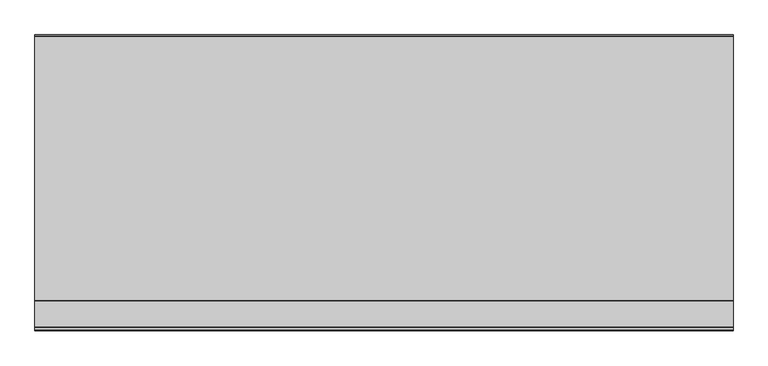
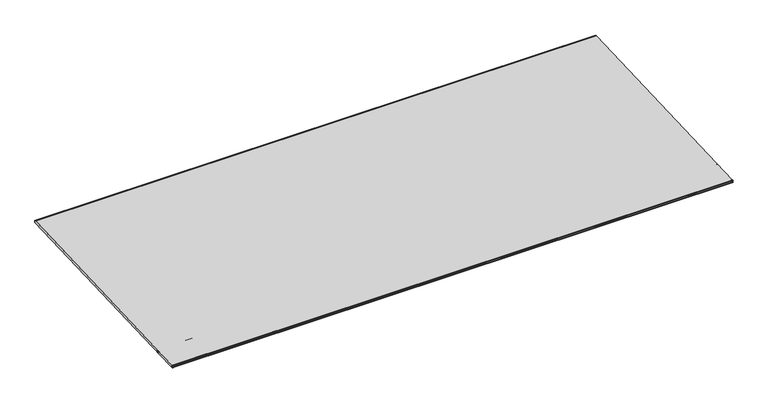
"""IFC4 building model written with IfcOpenShell, lengths in millimetres: proxy geometry, Generic Models 7:Generic Models 1:2:Generic Models 1:2 : Generic Models 7:Generic Models 1:337419:4 : Generic Models 7:Generic Models 1:2:Generic Models 1:2 : Generic Models 7:Generic Models 1:337419:306751."""

from ifc_helpers import new_model, si_unit, frame, origin, place, context, project, spatial, polyline, outline, extrude, source, transform, mapped, element, save


def generic_models_aa4b1cd0(model_context):
    return source(origin(), model_context, "Body", "SweptSolid", [
        extrude(outline(polyline([(-568149.1838193, 8805.2566863), (-568147.5976955, 8767.1897163), (-568071.3707252, 8770.36584), (-568072.956849, 8808.4328101), (-536698.3814292, 10115.7067859), (-536658.8157335, 10091.9333175), (-536560.4167528, 10096.0332751), (-536560.4167528, 9844.1294381), (-536557.2913841, 9844.2596618), (-536557.2913841, 9838.7653534), (-567628.0606235, 8544.1499684), (-567630.3076322, 8598.078176), (-567795.006937, 8591.215705), (-567792.6895197, 8535.5976883), (-568185.3148179, 8519.2383009), (-568185.3148179, 8572.9557309), (-568212.7692368, 8571.8117968), (-568212.7692368, 8573.8089425), (-568185.3148179, 8574.9528766), (-568185.3148179, 8762.5343219), (-568214.3718713, 8762.5343219), (-568214.3718713, 8802.5405175), (-568149.1838193, 8805.2566863)]), holes=[polyline([(-564954.3721269, 8702.0759872), (-564700.6374503, 8712.6482654), (-564700.9599621, 8720.3885493), (-564749.0565214, 8718.384526), (-564756.9659918, 8908.2118168), (-564709.1919444, 8910.2024022), (-564709.5250304, 8918.1964659), (-564962.9371952, 8907.6376257), (-564954.3721269, 8702.0759872)]), polyline([(-568181.3931281, 8575.1162804), (-568179.2782965, 8524.3603203), (-568014.5789916, 8531.2227913), (-568016.6938233, 8581.9787514), (-568181.3931281, 8575.1162804)])]), frame((591306.0367242, 0.0, 0.0), z_axis=(1.0, 0.0, 0.0), x_axis=(0.0, 1.0, 0.0)), (0.0, 0.0, 1.0), 74650.2368117),
    ])


if __name__ == "__main__":
    model = new_model("IFC4")
    model_context = context("Model", 3, world=origin())
    ifc_project = project(units=[si_unit("LENGTHUNIT", "METRE", prefix="MILLI")], contexts=[model_context])
    site = spatial("IfcSite", under=ifc_project)
    building = spatial("IfcBuilding", under=site)
    placement = place(None, origin())
    generic_models_shape = generic_models_aa4b1cd0(model_context)
    element("IfcBuildingElementProxy", 1, Name="Generic Models 7:Generic Models 1:2:Generic Models 1:2 : Generic Models 7:Generic Models 1:337419:4 : Generic Models 7:Generic Models 1:2:Generic Models 1:2 : Generic Models 7:Generic Models 1:337419:306751", ObjectType="Generic Models 7:Generic Models 1:2:Generic Models 1:2 : Generic Models 7:Generic Models 1:337419:4 : Generic Models 7:Generic Models 1:2:Generic Models 1:2 : Generic Models 7:Generic Models 1:337419:306751", at=placement, inside=building, context=model_context, shape_type="MappedRepresentation", body=[
        mapped(generic_models_shape, transform((0.0, 0.0, 0.0), x_axis=(1.0, 0.0, 0.0), y_axis=(0.0, 1.0, 0.0), z_axis=(0.0, 0.0, 1.0))),
    ])
    save(model, "model.ifc")

# Revit data of these elements
# Type "Generic Models 7:Generic Models 1:2:Generic Models 1:2 : Generic Models 7:Generic Models 1:337419:4 : Generic Models 7:Generic Models 1:2:Generic Models 1:2 : Generic Models 7:Generic Models 1:337419:306751"
#   NameOverride = "Generic Models 7:Generic Models 1:2:Generic Models 1:2 : Generic Models 7:Generic Models 1:337419:306751"
#   ObjectTypeOverride = "Generic Models 1:2 : Generic Models 7:Generic Models 1:337419"
#   Reference = "Generic Models 1"
#   Tag = "306751"
# Element 1 (IfcBuildingElementProxy, "Generic Models 7:Generic Models 1:2:Generic Models 1:2 : Generic Models 7:Generic Models 1:337419:4 : Generic Models 7:Generic Models 1:2:Generic Models 1:2 : Generic Models 7:Generic Models 1:337419:306751")
#   Materials on its faces: "CLASS A FIBERGLASS INSULATION WITH DURABLE VAPOR BARRIER (WHITE) LINE"
# Materials
#   "CLASS A FIBERGLASS INSULATION WITH DURABLE VAPOR BARRIER (WHITE) LINE": class "Unassigned", colour RGB 187 139 199, transparency 0, Cost = 0
